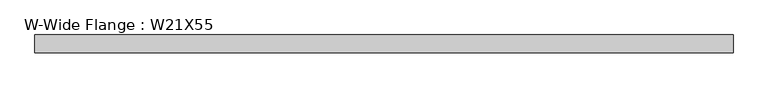
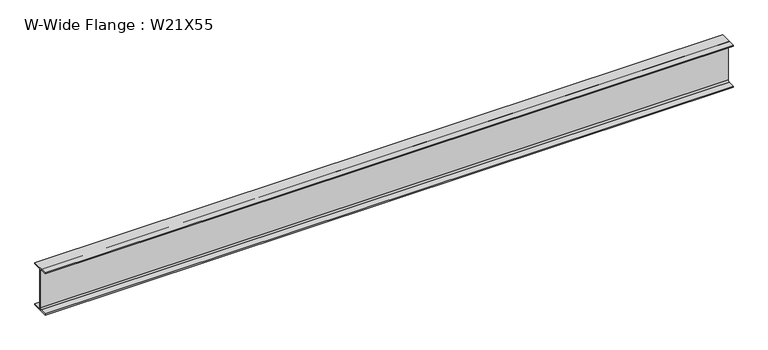
"""IFC4 building model written with IfcOpenShell, lengths in millimetres: beam geometry, W-Wide Flange : W21X55."""

import ifcopenshell
import ifcopenshell.guid

model = None  # the IFC model being written
_history = None  # IfcOwnerHistory: only IFC2X3 demands one
_inside = {}  # id of a spatial element -> (the spatial element, [elements in it])
_under = {}  # id of a project, library or spatial element -> (it, [spatial elements below it])
_declared = {}  # id of a project -> (the project, [libraries it declares])
_typed = {}  # id of a type object -> (the type object, [elements of that type])
_made_of = {}  # id of a material, layer set ... -> (it, [elements and type objects made of it])


def new_model(schema):
    """Start an empty IFC model of exactly this schema.

    Asked for "IFC4X3", IfcOpenShell would pick the latest addendum, in which some entities
    have other attributes; the version numbers below select the first issue.
    IFC2X3 requires an IfcOwnerHistory on every rooted entity: one is made here for all.
    """
    global model, _history
    if schema == "IFC4X3":
        model = ifcopenshell.file(schema_version=(4, 3, 0, 0))
    else:
        model = ifcopenshell.file(schema=schema)
    _inside.clear()
    _under.clear()
    _declared.clear()
    _typed.clear()
    _made_of.clear()
    _history = None
    if model.schema == "IFC2X3":
        org = make("IfcOrganization", Name="unknown")
        user = make(
            "IfcPersonAndOrganization",
            ThePerson=make("IfcPerson", FamilyName="unknown"),
            TheOrganization=org,
        )
        app = make(
            "IfcApplication",
            ApplicationDeveloper=org,
            Version="unknown",
            ApplicationFullName="unknown",
            ApplicationIdentifier="unknown",
        )
        _history = make(
            "IfcOwnerHistory",
            OwningUser=user,
            OwningApplication=app,
            ChangeAction="ADDED",
            CreationDate=0,
        )
    return model


def make(cls, **values):
    """One entity of the class cls with the attributes given. An attribute that is None is left unset."""
    return model.create_entity(
        cls, **{name: value for name, value in values.items() if value is not None}
    )


def rooted(cls, **values):
    """An entity with a GlobalId (a new one), such as an element, a storey or a relation."""
    return make(cls, GlobalId=ifcopenshell.guid.new(), OwnerHistory=_history, **values)


def si_unit(unit_type, name, prefix=None):
    """IfcSIUnit, for example si_unit("LENGTHUNIT", "METRE", prefix="MILLI")."""
    return make("IfcSIUnit", UnitType=unit_type, Prefix=prefix, Name=name)


def assignment(units):
    """IfcUnitAssignment: the units of a project."""
    return None if units is None else make("IfcUnitAssignment", Units=units)


def point(xyz):
    """IfcCartesianPoint."""
    return None if xyz is None else make("IfcCartesianPoint", Coordinates=xyz)


def direction(xyz):
    """IfcDirection."""
    return None if xyz is None else make("IfcDirection", DirectionRatios=xyz)


def frame(location, z_axis=None, x_axis=None):
    """IfcAxis2Placement3D, a coordinate frame: its origin and axes. An axis left out is left unset."""
    return make(
        "IfcAxis2Placement3D",
        Location=point(location),
        Axis=direction(z_axis),
        RefDirection=direction(x_axis),
    )


def frame_2d(location, x_axis=None):
    """IfcAxis2Placement2D, a coordinate frame in the plane: its origin and x axis."""
    return make(
        "IfcAxis2Placement2D", Location=point(location), RefDirection=direction(x_axis)
    )


def origin():
    """The frame at (0, 0, 0) with its axes left unset."""
    return frame((0.0, 0.0, 0.0))


def place(relative_to, where):
    """IfcLocalPlacement: puts the frame where relative to a parent placement (None: the world)."""
    return make(
        "IfcLocalPlacement", PlacementRelTo=relative_to, RelativePlacement=where
    )


def context(
    kind, dimensions, precision=None, world=None, true_north=None, identifier=None
):
    """IfcGeometricRepresentationContext, for example the 3D "Model" context."""
    return make(
        "IfcGeometricRepresentationContext",
        ContextIdentifier=identifier,
        ContextType=kind,
        CoordinateSpaceDimension=dimensions,
        Precision=precision,
        WorldCoordinateSystem=world,
        TrueNorth=true_north,
    )


def project(units=None, contexts=None):
    """IfcProject with its units and contexts."""
    return rooted(
        "IfcProject",
        Name="project",
        RepresentationContexts=contexts,
        UnitsInContext=assignment(units),
    )


def spatial(cls, under=None, at=None, **own):
    """A site, building, storey or space (cls), placed at a placement, below another one or the project."""
    s = rooted(cls, ObjectPlacement=at, **own)
    if under is not None:
        _under.setdefault(under.id(), (under, []))[1].append(s)
    return s


def polyline(points):
    """IfcPolyline through the points."""
    return make("IfcPolyline", Points=[point(p) for p in points])


def circle_curve(where, radius):
    """IfcCircle in the frame where."""
    return make("IfcCircle", Position=where, Radius=radius)


def trimmed(basis, trim1, trim2, sense, master):
    """IfcTrimmedCurve: the piece of a basis curve between two trims."""
    return make(
        "IfcTrimmedCurve",
        BasisCurve=basis,
        Trim1=trim1,
        Trim2=trim2,
        SenseAgreement=sense,
        MasterRepresentation=master,
    )


def segment(curve, same_sense, transition):
    """IfcCompositeCurveSegment."""
    return make(
        "IfcCompositeCurveSegment",
        Transition=transition,
        SameSense=same_sense,
        ParentCurve=curve,
    )


def composite_curve(segments, self_intersect=None):
    """IfcCompositeCurve: segments joined end to end."""
    return make("IfcCompositeCurve", Segments=segments, SelfIntersect=self_intersect)


def outline(outer, holes=None, kind="AREA"):
    """IfcArbitraryClosedProfileDef: a profile drawn as a closed curve; with holes, ...WithVoids."""
    if holes is None:
        return make("IfcArbitraryClosedProfileDef", ProfileType=kind, OuterCurve=outer)
    return make(
        "IfcArbitraryProfileDefWithVoids",
        ProfileType=kind,
        OuterCurve=outer,
        InnerCurves=holes,
    )


def extrude(swept, where, along, depth):
    """IfcExtrudedAreaSolid: the profile swept, set in the frame where, extruded along a direction by depth."""
    return make(
        "IfcExtrudedAreaSolid",
        SweptArea=swept,
        Position=where,
        ExtrudedDirection=direction(along),
        Depth=depth,
    )


def shape(context_of_items, identifier, shape_type, items):
    """IfcShapeRepresentation: the items that make up one representation, for example the "Body"."""
    return make(
        "IfcShapeRepresentation",
        ContextOfItems=context_of_items,
        RepresentationIdentifier=identifier,
        RepresentationType=shape_type,
        Items=items,
    )


def source(mapping_origin, context_of_items, identifier, shape_type, items):
    """IfcRepresentationMap: a shape defined once, which mapped items show again and again."""
    return make(
        "IfcRepresentationMap",
        MappingOrigin=mapping_origin,
        MappedRepresentation=shape(context_of_items, identifier, shape_type, items),
    )


def transform(
    local_origin,
    x_axis=None,
    y_axis=None,
    z_axis=None,
    scale=None,
    scale2=None,
    scale3=None,
    uniform=True,
):
    """IfcCartesianTransformationOperator3D, or its non-uniform kind. x_axis, y_axis, z_axis: its Axis1, 2, 3."""
    if uniform:
        return make(
            "IfcCartesianTransformationOperator3D",
            Axis1=direction(x_axis),
            Axis2=direction(y_axis),
            LocalOrigin=point(local_origin),
            Scale=scale,
            Axis3=direction(z_axis),
        )
    return make(
        "IfcCartesianTransformationOperator3DnonUniform",
        Axis1=direction(x_axis),
        Axis2=direction(y_axis),
        LocalOrigin=point(local_origin),
        Scale=scale,
        Axis3=direction(z_axis),
        Scale2=scale2,
        Scale3=scale3,
    )


def mapped(mapping_source, mapping_target):
    """IfcMappedItem: shows the shape of a source again, moved by a transform."""
    return make(
        "IfcMappedItem", MappingSource=mapping_source, MappingTarget=mapping_target
    )


def made_of(thing, what):
    """Note that an element or type object is made of a material, layer set ...; save() writes the relation."""
    if what is not None:
        _made_of.setdefault(what.id(), (what, []))[1].append(thing)
    return thing


def element(
    cls,
    number,
    at=None,
    inside=None,
    cuts=None,
    type_object=None,
    material=None,
    context=None,
    identifier="Body",
    shape_type=None,
    held_by="IfcProductDefinitionShape",
    body=None,
    shapes=None,
    **own,
):
    """One element of the class cls, such as IfcWall. Its Tag is "e" and its number.

    at: its placement. inside: the storey or other place that contains it. cuts: it is an
    opening in that element (IfcRelVoidsElement). A single representation is given by context,
    identifier, shape_type and body (its items); several are given by shapes. held_by: the class
    of the entity that holds the representations. save() writes the other relations.
    """
    e = rooted(cls, Tag="e%d" % number, ObjectPlacement=at, **own)
    if body is not None:
        shapes = [shape(context, identifier, shape_type, body)]
    if shapes is not None:
        e.Representation = make(held_by, Representations=shapes)
    if inside is not None:
        _inside.setdefault(inside.id(), (inside, []))[1].append(e)
    if cuts is not None:
        rooted(
            "IfcRelVoidsElement", RelatingBuildingElement=cuts, RelatedOpeningElement=e
        )
    if type_object is not None:
        _typed.setdefault(type_object.id(), (type_object, []))[1].append(e)
    return made_of(e, material)


def aggregate(whole, parts):
    """IfcRelAggregates: a whole, such as a stair, and the parts it consists of."""
    return rooted("IfcRelAggregates", RelatingObject=whole, RelatedObjects=parts)


def save(model, path):
    """Write the relations noted so far, then the file.

    IfcRelAggregates (storeys below a building ...), IfcRelContainedInSpatialStructure (elements
    in a storey), IfcRelDefinesByType, IfcRelAssociatesMaterial and IfcRelDeclares: one each for
    every whole, place, type object, material and project.
    """
    for whole, parts in _under.values():
        aggregate(whole, parts)
    for where, things in _inside.values():
        rooted(
            "IfcRelContainedInSpatialStructure",
            RelatedElements=things,
            RelatingStructure=where,
        )
    for kind, things in _typed.values():
        rooted("IfcRelDefinesByType", RelatedObjects=things, RelatingType=kind)
    for what, things in _made_of.values():
        rooted("IfcRelAssociatesMaterial", RelatedObjects=things, RelatingMaterial=what)
    for by, libraries in _declared.values():
        rooted("IfcRelDeclares", RelatingContext=by, RelatedDefinitions=libraries)
    model.write(path)


def w_wide_flange_w21x55_637cb683(model_context):
    return source(origin(), model_context, "Body", "SweptSolid", [
        extrude(outline(composite_curve([segment(polyline([(104.394, -250.9012), (104.394, -264.16), (-104.394, -264.16), (-104.394, -250.9012), (-21.6662, -250.9012)]), True, "CONTINUOUS"), segment(trimmed(circle_curve(frame_2d((-21.6662, -233.9975)), 16.9037), [point((-21.6662, -250.9012))], [point((-4.7625, -233.9975))], True, "CARTESIAN"), True, "CONTINUOUS"), segment(polyline([(-4.7625, -233.9975), (-4.7625, 233.9975)]), True, "CONTINUOUS"), segment(trimmed(circle_curve(frame_2d((-21.6662, 233.9975)), 16.9037), [point((-4.7625, 233.9975))], [point((-21.6662, 250.9012))], True, "CARTESIAN"), True, "CONTINUOUS"), segment(polyline([(-21.6662, 250.9012), (-104.394, 250.9012), (-104.394, 264.16), (104.394, 264.16), (104.394, 250.9012), (21.6662, 250.9012)]), True, "CONTINUOUS"), segment(trimmed(circle_curve(frame_2d((21.6662, 233.9975)), 16.9037), [point((21.6662, 250.9012))], [point((4.7625, 233.9975))], True, "CARTESIAN"), True, "CONTINUOUS"), segment(polyline([(4.7625, 233.9975), (4.7625, -233.9975)]), True, "CONTINUOUS"), segment(trimmed(circle_curve(frame_2d((21.6662, -233.9975)), 16.9037), [point((4.7625, -233.9975))], [point((21.6662, -250.9012))], True, "CARTESIAN"), True, "CONTINUOUS"), segment(polyline([(21.6662, -250.9012), (104.394, -250.9012)]), True, "CONTINUOUS")], self_intersect=False)), frame((-4076.7, 0.0, 0.0), z_axis=(1.0, 0.0, 0.0), x_axis=(0.0, 1.0, 0.0)), (0.0, 0.0, 1.0), 8153.4),
    ])


if __name__ == "__main__":
    model = new_model("IFC4")
    model_context = context("Model", 3, world=origin())
    ifc_project = project(units=[si_unit("LENGTHUNIT", "METRE", prefix="MILLI")], contexts=[model_context])
    site = spatial("IfcSite", under=ifc_project)
    building = spatial("IfcBuilding", under=site)
    placement = place(None, origin())
    w_wide_flange_w21x55_shape = w_wide_flange_w21x55_637cb683(model_context)
    element("IfcBeam", 1, ObjectType="W-Wide Flange : W21X55", at=placement, inside=building, context=model_context, shape_type="MappedRepresentation", body=[
        mapped(w_wide_flange_w21x55_shape, transform((0.0, 0.0, 0.0), x_axis=(1.0, 0.0, 0.0), y_axis=(0.0, 1.0, 0.0), z_axis=(0.0, 0.0, 1.0))),
    ])
    save(model, "model.ifc")

# Revit data of these elements
# Type "W-Wide Flange : W21X55"
#   Assembly Code = "B10"
#   W = 55
#   Length [instance default] = 5' - 0"
#   bf = 0' - 8.22"
#   d = 1' - 8.8"
#   k = 0' - 1 3/16"
#   k2 = 0' - 0.6655"
#   tf = 0' - 0.522"
#   tw = 0' - 0 3/8"
#   A = 0.1125 SF
#   Structural Material [instance default] = Steel ASTM A992
# Element 1 (IfcBeam, "W-Wide Flange : W21X55")
#   Materials on its faces: "Steel ASTM A992"
# Materials
#   "Steel ASTM A992": class "Metal", colour RGB 199 199 199, transparency 0, Description = "Structural steel 50ksi", Cost = 0
